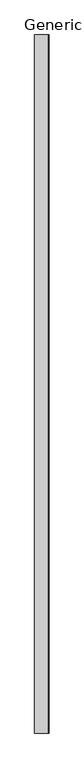
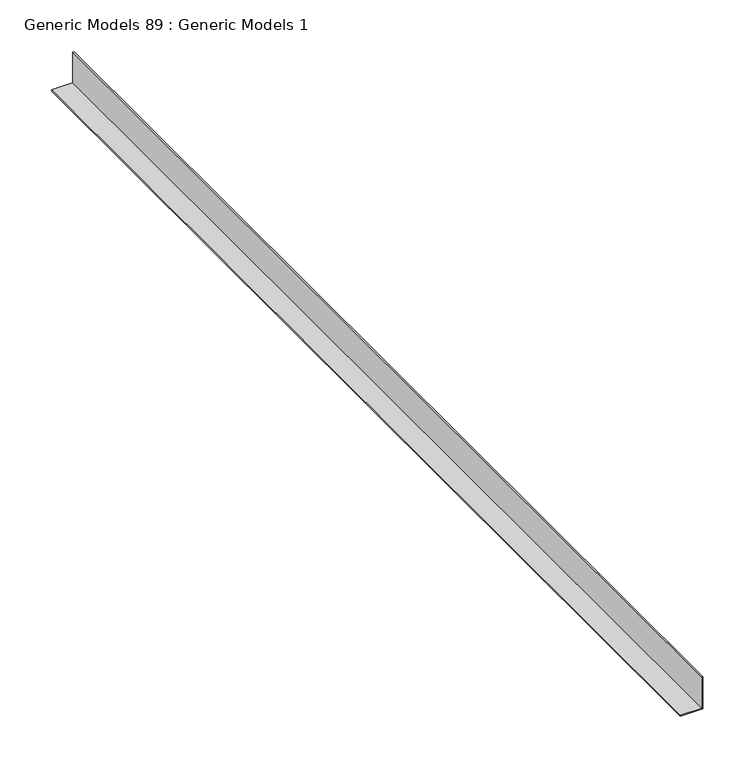
"""IFC4 building model written with IfcOpenShell, lengths in millimetres: proxy geometry, Generic Models 89 : Generic Models 1."""

from ifc_helpers import new_model, si_unit, frame, origin, place, context, project, spatial, polyline, outline, extrude, source, transform, mapped, element, save


def generic_models_89_generic_models_1_217c0eea(model_context):
    return source(origin(), model_context, "Body", "SweptSolid", [
        extrude(outline(polyline([(2304.9709098, 49676.05), (2304.9709098, 49674.4625), (2268.4584098, 49674.4625), (2268.4584098, 49650.65), (2266.8709098, 49650.65), (2266.8709098, 49676.05), (2304.9709098, 49676.05)])), frame((0.0, 0.0, 0.0), z_axis=(0.0, 1.0, 0.0), x_axis=(0.0, 0.0, 1.0)), (0.0, 0.0, 1.0), 1219.2),
    ])


if __name__ == "__main__":
    model = new_model("IFC4")
    model_context = context("Model", 3, world=origin())
    ifc_project = project(units=[si_unit("LENGTHUNIT", "METRE", prefix="MILLI")], contexts=[model_context])
    site = spatial("IfcSite", under=ifc_project)
    building = spatial("IfcBuilding", under=site)
    placement = place(None, origin())
    generic_models_89_generic_models_1_shape = generic_models_89_generic_models_1_217c0eea(model_context)
    element("IfcBuildingElementProxy", 1, Name="Generic Models 89 : Generic Models 1", ObjectType="Generic Models 89 : Generic Models 1", at=placement, inside=building, context=model_context, shape_type="MappedRepresentation", body=[
        mapped(generic_models_89_generic_models_1_shape, transform((0.0, 0.0, 0.0), x_axis=(1.0, 0.0, 0.0), y_axis=(0.0, 1.0, 0.0), z_axis=(0.0, 0.0, 1.0))),
    ])
    save(model, "model.ifc")

# Revit data of these elements
# Element 1 (IfcBuildingElementProxy, "Generic Models 89 : Generic Models 1")
#   Materials on its faces: "CEILING TRACK AS SCHEDULED"
# Materials
#   "CEILING TRACK AS SCHEDULED": class "Unassigned", colour RGB 210 209 208, transparency 0, Keynote = "M05121300.02", Cost = 0
